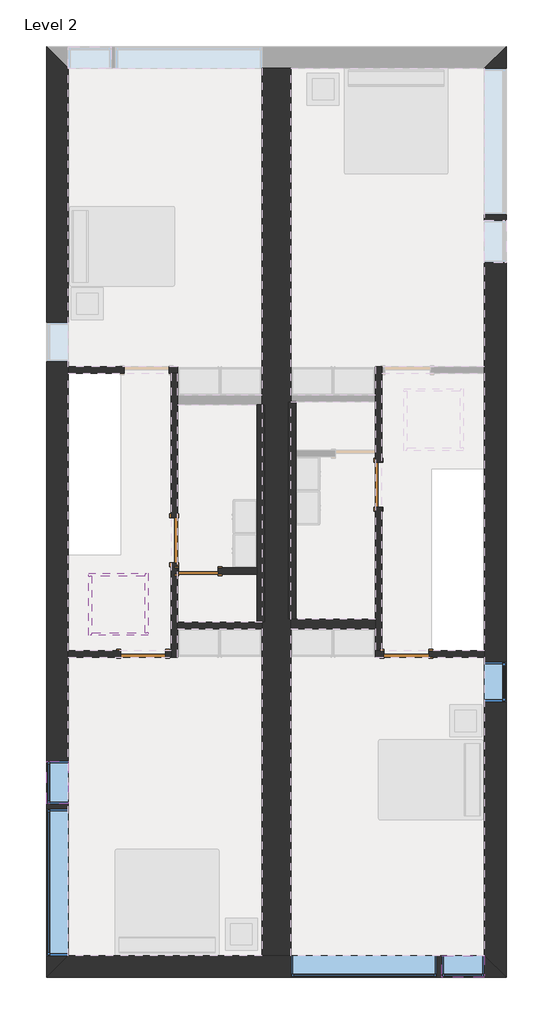
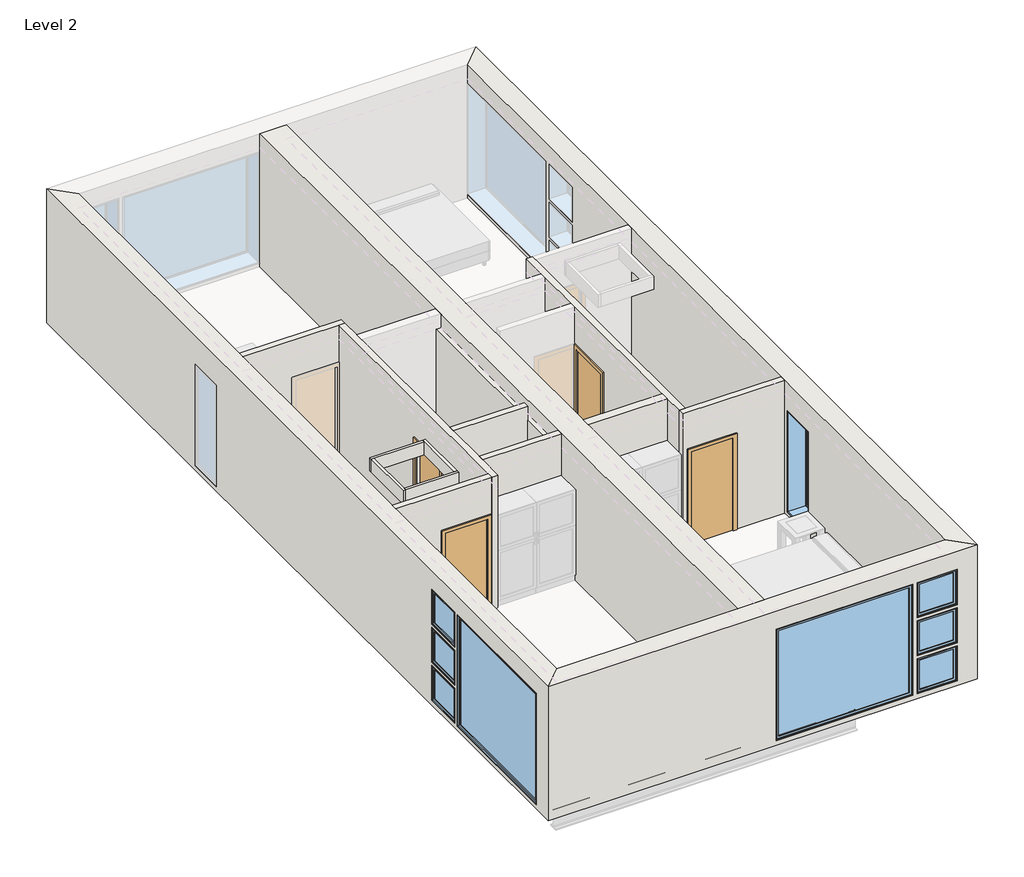
# One storey, part 1 of 2: 20 walls, 9 windows, 5 doors.
# Revit data of these elements (continued)
# Type "Interior - Partition (92mm Stud)" (continued)
#   Constituents = "Constituents"
#   Features = "Features"
#   Finish = "Finish"
#   Grade = "Grade"
#   Material = "Material"
#   ModelReference = "ModelReference"
#   NominalHeight = "NominalHeight"
#   NominalLength = "NominalLength"
#   NominalWidth = "NominalWidth"
#   ProductionYear = "ProductionYear"
#   Reference = "Reference"
#   Shape = "Shape"
#   Size = "Size"
#   SustainabilityPerformance = "SustainabilityPerformance"
#   WarrantyDescription = "WarrantyDescription"
#   WarrantyDurationLabor = "WarrantyDurationLabor"
#   WarrantyDurationParts = "WarrantyDurationParts"
#   WarrantyGuarantorLabor = "WarrantyGuarantorLabor"
#   WarrantyGuarantorParts = "WarrantyGuarantorParts"
#   ExpectedLife = "ExpectedLife"
#   ReplacementCost = "ReplacementCost"
#   AssetAccountingType = "FIXED"
#   Classification Description = "Metal-Framed Gypsum Board Fixed Partitions"
#   Classification Code = "23-25 40 11 11 11"
#   ModelLabel = "ModelLabel"
#   Layers, outside or top first: 0.016 m "Plasterboard" (function 5); 0.092 m "Metal - Stud Layer" (function 1); 0.016 m "Plasterboard" (function 5)
# Type "Interior - Plumbing (152mm Stud)"
#   Manufacturer = "Manufacturer"
#   AccessibilityPerformance = "AccessibilityPerformance"
#   CodePerformance = "CodePerformance"
#   Color = "Color"
#   Constituents = "Constituents"
#   Features = "Features"
#   Finish = "Finish"
#   Grade = "Grade"
#   Material = "Material"
#   ModelReference = "ModelReference"
#   NominalHeight = "NominalHeight"
#   NominalLength = "NominalLength"
#   NominalWidth = "NominalWidth"
#   ProductionYear = "ProductionYear"
#   Reference = "Reference"
#   Shape = "Shape"
#   Size = "Size"
#   SustainabilityPerformance = "SustainabilityPerformance"
#   WarrantyDescription = "WarrantyDescription"
#   WarrantyDurationLabor = "WarrantyDurationLabor"
#   WarrantyDurationParts = "WarrantyDurationParts"
#   WarrantyGuarantorLabor = "WarrantyGuarantorLabor"
#   WarrantyGuarantorParts = "WarrantyGuarantorParts"
#   ExpectedLife = "ExpectedLife"
#   ReplacementCost = "ReplacementCost"
#   AssetAccountingType = "FIXED"
#   Classification Description = "Metal-Framed Gypsum Board Fixed Partitions"
#   Classification Code = "23-25 40 11 11 11"
#   ModelLabel = "ModelLabel"
#   Layers, outside or top first: 0.016 m "Plasterboard" (function 5); 0.152 m "Metal - Stud Layer" (function 1); 0.016 m "Plasterboard" (function 5)
# Type "M_Casement : 819mm x 759mm"
#   Manufacturer = "Manufacturer"
#   Type Mark = "03"
#   Construction Type = "Construction Type"
#   AccessibilityPerformance = "AccessibilityPerformance"
#   CodePerformance = "CodePerformance"
#   ConfigurationType = "ConfigurationType"
#   ConstructionType = "ConstructionType"
#   FireRating = "FireRating"
#   GlazingAreaFraction = "GlazingAreaFraction"
#   OperationType = "OperationType"
#   Area = "Area"
#   Color = "Color"
#   Constituents = "Constituents"
#   Features = "Features"
#   Finish = "Finish"
#   Grade = "Grade"
#   Material = "Material"
#   ModelReference = "ModelReference"
#   NominalHeight = "NominalHeight"
#   NominalLength = "NominalLength"
#   NominalWidth = "NominalWidth"
#   ProductionYear = "ProductionYear"
#   Reference = "Reference"
#   Shape = "Shape"
#   Size = "Size"
#   SustainabilityPerformance = "SustainabilityPerformance"
#   WarrantyDescription = "WarrantyDescription"
#   WarrantyDurationLabor = "WarrantyDurationLabor"
#   WarrantyDurationParts = "WarrantyDurationParts"
#   WarrantyGuarantorLabor = "WarrantyGuarantorLabor"
#   WarrantyGuarantorParts = "WarrantyGuarantorParts"
#   ExpectedLife = "ExpectedLife"
#   ReplacementCost = "ReplacementCost"
#   AssetAccountingType = "FIXED"
#   ModelLabel = "ModelLabel"
#   Height = 0.759 m
#   Default Sill Height = 0.915 m
#   Width = 0.819 m
#   Window Inset = 0.019 m
#   Glass Pane Material = Glass
#   Sash = Sash
#   Trim Exterior Material = Trim
#   Trim Interior Material = Trim
#   Wall Closure = (empty or 0)
# Type "M_Fixed : 2800mm x 2410mm"
#   Manufacturer = "Manufacturer"
#   Type Mark = "01"
#   Construction Type = "Construction Type"
#   AccessibilityPerformance = "AccessibilityPerformance"
#   CodePerformance = "CodePerformance"
#   ConfigurationType = "ConfigurationType"
#   ConstructionType = "ConstructionType"
#   FireRating = "FireRating"
#   GlazingAreaFraction = "GlazingAreaFraction"
#   OperationType = "OperationType"
#   Area = "Area"
#   Color = "Color"
#   Constituents = "Constituents"
#   Features = "Features"
#   Finish = "Finish"
#   Grade = "Grade"
#   Material = "Material"
#   ModelReference = "ModelReference"
#   NominalHeight = "NominalHeight"
#   NominalLength = "NominalLength"
#   NominalWidth = "NominalWidth"
#   ProductionYear = "ProductionYear"
#   Reference = "Reference"
#   Shape = "Shape"
#   Size = "Size"
#   SustainabilityPerformance = "SustainabilityPerformance"
#   WarrantyDescription = "WarrantyDescription"
#   WarrantyDurationLabor = "WarrantyDurationLabor"
#   WarrantyDurationParts = "WarrantyDurationParts"
#   WarrantyGuarantorLabor = "WarrantyGuarantorLabor"
#   WarrantyGuarantorParts = "WarrantyGuarantorParts"
#   ExpectedLife = "ExpectedLife"
#   ReplacementCost = "ReplacementCost"
#   AssetAccountingType = "FIXED"
#   ModelLabel = "ModelLabel"
#   Height = 2.410 m
#   Default Sill Height = 0.100 m
#   Width = 2.800 m
#   Window Inset = 0.019 m
#   Frame Exterior Material = Sash
#   Frame Interior Material = Sash
#   Glass Pane Material = Glass
#   Sash = Sash
#   Wall Closure = (empty or 0)
# Type "M_Fixed : 750mm x 2200mm"
#   Manufacturer = "Manufacturer"
#   Type Mark = "04"
#   Construction Type = "Construction Type"
#   AccessibilityPerformance = "AccessibilityPerformance"
#   CodePerformance = "CodePerformance"
#   ConfigurationType = "ConfigurationType"
#   ConstructionType = "ConstructionType"
#   FireRating = "FireRating"
#   GlazingAreaFraction = "GlazingAreaFraction"
#   OperationType = "OperationType"
#   Area = "Area"
#   Color = "Color"
#   Constituents = "Constituents"
#   Features = "Features"
#   Finish = "Finish"
#   Grade = "Grade"
#   Material = "Material"
#   ModelReference = "ModelReference"
#   NominalHeight = "NominalHeight"
#   NominalLength = "NominalLength"
#   NominalWidth = "NominalWidth"
#   ProductionYear = "ProductionYear"
#   Reference = "Reference"
#   Shape = "Shape"
#   Size = "Size"
#   SustainabilityPerformance = "SustainabilityPerformance"
#   WarrantyDescription = "WarrantyDescription"
#   WarrantyDurationLabor = "WarrantyDurationLabor"
#   WarrantyDurationParts = "WarrantyDurationParts"
#   WarrantyGuarantorLabor = "WarrantyGuarantorLabor"
#   WarrantyGuarantorParts = "WarrantyGuarantorParts"
#   ExpectedLife = "ExpectedLife"
#   ReplacementCost = "ReplacementCost"
#   AssetAccountingType = "FIXED"
#   ModelLabel = "ModelLabel"
#   Height = 2.200 m
#   Default Sill Height = 0.100 m
#   Width = 0.750 m
#   Window Inset = 0.019 m
#   Frame Exterior Material = Sash
#   Frame Interior Material = Sash
#   Glass Pane Material = Glass
#   Sash = Sash
#   Wall Closure = (empty or 0)
# Type "M_Fixed : 819mm x 759mm"
#   Manufacturer = "Manufacturer"
#   Type Mark = "02"
#   Construction Type = "Construction Type"
#   AccessibilityPerformance = "AccessibilityPerformance"
#   CodePerformance = "CodePerformance"
#   ConfigurationType = "ConfigurationType"
#   ConstructionType = "ConstructionType"
#   FireRating = "FireRating"
#   GlazingAreaFraction = "GlazingAreaFraction"
#   OperationType = "OperationType"
#   Area = "Area"
#   Color = "Color"
#   Constituents = "Constituents"
#   Features = "Features"
#   Finish = "Finish"
#   Grade = "Grade"
#   Material = "Material"
#   ModelReference = "ModelReference"
#   NominalHeight = "NominalHeight"
#   NominalLength = "NominalLength"
#   NominalWidth = "NominalWidth"
#   ProductionYear = "ProductionYear"
#   Reference = "Reference"
#   Shape = "Shape"
#   Size = "Size"
#   SustainabilityPerformance = "SustainabilityPerformance"
#   WarrantyDescription = "WarrantyDescription"
#   WarrantyDurationLabor = "WarrantyDurationLabor"
#   WarrantyDurationParts = "WarrantyDurationParts"
#   WarrantyGuarantorLabor = "WarrantyGuarantorLabor"
#   WarrantyGuarantorParts = "WarrantyGuarantorParts"
#   ExpectedLife = "ExpectedLife"
#   ReplacementCost = "ReplacementCost"
#   AssetAccountingType = "FIXED"
#   ModelLabel = "ModelLabel"
#   Height = 0.759 m
#   Default Sill Height = 0.100 m
#   Width = 0.819 m
#   Window Inset = 0.019 m
#   Frame Exterior Material = Sash
#   Frame Interior Material = Sash
#   Glass Pane Material = Glass
#   Sash = Sash
#   Wall Closure = (empty or 0)
# Element 1 (IfcDoor, "M_Single-Flush : 0762 x 2032mm")
#   InstallationDate = "InstallationDate"
#   SerialNumber = "SerialNumber"
#   WarrantyStartDate = "WarrantyStartDate"
#   BarCode = "BarCode"
#   AssetIdentifier = "AssetIdentifier"
#   TagNumber = "TagNumber"
#   URI = "https://niras.dk/projects/0001/door_1xS3BCk291UvhgP2dvNd%24j"
#   Phase Created = New Construction
#   Materials on its faces: "Door - Frame", "Door - Panel"
# Element 2 (IfcDoor, "M_Single-Flush : 0864 x 2032mm")
#   InstallationDate = "InstallationDate"
#   SerialNumber = "SerialNumber"
#   WarrantyStartDate = "WarrantyStartDate"
#   BarCode = "BarCode"
#   AssetIdentifier = "AssetIdentifier"
#   TagNumber = "TagNumber"
#   URI = "https://niras.dk/projects/0001/door_1xS3BCk291UvhgP2dvNo%24h"
#   Phase Created = New Construction
#   Materials on its faces: "Door - Frame", "Door - Panel"
# Element 3 (IfcDoor, "M_Single-Flush : 0864 x 2032mm")
#   InstallationDate = "InstallationDate"
#   SerialNumber = "SerialNumber"
#   WarrantyStartDate = "WarrantyStartDate"
#   BarCode = "BarCode"
#   AssetIdentifier = "AssetIdentifier"
#   TagNumber = "TagNumber"
#   URI = "https://niras.dk/projects/0001/door_1xS3BCk291UvhgP2dvNnLa"
#   Phase Created = New Construction
#   Materials on its faces: "Door - Frame", "Door - Panel"
# Element 4 (IfcDoor, "M_Single-Flush : 0864 x 2032mm")
#   InstallationDate = "InstallationDate"
#   SerialNumber = "SerialNumber"
#   WarrantyStartDate = "WarrantyStartDate"
#   BarCode = "BarCode"
#   AssetIdentifier = "AssetIdentifier"
#   TagNumber = "TagNumber"
#   URI = "https://niras.dk/projects/0001/door_1xS3BCk291UvhgP2dvNnNr"
#   Phase Created = New Construction
#   Materials on its faces: "Door - Frame", "Door - Panel"
# Element 5 (IfcDoor, "M_Single-Flush : 0864 x 2032mm")
#   InstallationDate = "InstallationDate"
#   SerialNumber = "SerialNumber"
#   WarrantyStartDate = "WarrantyStartDate"
#   BarCode = "BarCode"
#   AssetIdentifier = "AssetIdentifier"
#   TagNumber = "TagNumber"
#   URI = "https://niras.dk/projects/0001/door_1xS3BCk291UvhgP2dvNmlJ"
#   Phase Created = New Construction
#   Materials on its faces: "Door - Frame", "Door - Panel"
# Element 6 (IfcWall, "Party Wall - CMU Residential Unit Dimising Wall")
#   InstallationDate = "InstallationDate"
#   SerialNumber = "SerialNumber"
#   WarrantyStartDate = "WarrantyStartDate"
#   BarCode = "BarCode"
#   AssetIdentifier = "AssetIdentifier"
#   TagNumber = "TagNumber"
#   URI = "https://niras.dk/projects/0001/wall_1xS3BCk291UvhgP2dvNqkY"
#   Top Offset = 0.000 m
#   Base Offset = 0.000 m
#   wall height = 2.900 m
#   Phase Created = New Construction
#   Base Constraint = Level 2
#   Top Constraint = Roof
#   Materials on its faces: "Default Wall", "Plasterboard"
# Element 7 (IfcWall, "Exterior - Brick on Block")
#   InstallationDate = "InstallationDate"
#   SerialNumber = "SerialNumber"
#   WarrantyStartDate = "WarrantyStartDate"
#   BarCode = "BarCode"
#   AssetIdentifier = "AssetIdentifier"
#   TagNumber = "TagNumber"
#   URI = "https://niras.dk/projects/0001/wall_1xS3BCk291UvhgP2dvNrHJ"
#   Top Offset = 0.000 m
#   Base Offset = 0.000 m
#   wall height = 2.900 m
#   Phase Created = New Construction
#   Base Constraint = Level 2
#   Top Constraint = Roof
#   Materials on its faces: "Default Wall", "Plasterboard", "Masonry - Brick"
# Element 8 (IfcWall, "Exterior - Brick on Block")
#   InstallationDate = "InstallationDate"
#   SerialNumber = "SerialNumber"
#   WarrantyStartDate = "WarrantyStartDate"
#   BarCode = "BarCode"
#   AssetIdentifier = "AssetIdentifier"
#   TagNumber = "TagNumber"
#   URI = "https://niras.dk/projects/0001/wall_1xS3BCk291UvhgP2dvNrIB"
#   Top Offset = 0.000 m
#   Base Offset = 0.000 m
#   wall height = 2.900 m
#   Phase Created = New Construction
#   Base Constraint = Level 2
#   Top Constraint = Roof
#   Materials on its faces: "Default Wall", "Plasterboard", "Masonry - Brick"
# Element 9 (IfcWall, "Exterior - Brick on Block")
#   InstallationDate = "InstallationDate"
#   SerialNumber = "SerialNumber"
#   WarrantyStartDate = "WarrantyStartDate"
#   BarCode = "BarCode"
#   AssetIdentifier = "AssetIdentifier"
#   TagNumber = "TagNumber"
#   URI = "https://niras.dk/projects/0001/wall_1xS3BCk291UvhgP2dvNrJ3"
#   Top Offset = 0.000 m
#   Base Offset = 0.000 m
#   wall height = 2.900 m
#   Phase Created = New Construction
#   Base Constraint = Level 2
#   Top Constraint = Roof
#   Materials on its faces: "Default Wall", "Plasterboard", "Masonry - Brick"
# Element 10 (IfcWall, "Interior - Furring (152 mm Stud)")
#   InstallationDate = "InstallationDate"
#   SerialNumber = "SerialNumber"
#   WarrantyStartDate = "WarrantyStartDate"
#   BarCode = "BarCode"
#   AssetIdentifier = "AssetIdentifier"
#   TagNumber = "TagNumber"
#   URI = "https://niras.dk/projects/0001/wall_1xS3BCk291UvhgP2dvNvRw"
#   Top Offset = -0.305 m
#   Base Offset = 0.000 m
#   wall height = 2.595 m
#   Phase Created = New Construction
#   Base Constraint = Level 2
#   Top Constraint = Roof
#   Materials on its faces: "Default Wall", "Metal - Stud Layer", "Plasterboard"
# Element 11 (IfcWall, "Interior - Furring (152 mm Stud)")
#   InstallationDate = "InstallationDate"
#   SerialNumber = "SerialNumber"
#   WarrantyStartDate = "WarrantyStartDate"
#   BarCode = "BarCode"
#   AssetIdentifier = "AssetIdentifier"
#   TagNumber = "TagNumber"
#   URI = "https://niras.dk/projects/0001/wall_1xS3BCk291UvhgP2dvNv9J"
#   Top Offset = -0.305 m
#   Base Offset = 0.000 m
#   wall height = 2.595 m
#   Phase Created = New Construction
#   Base Constraint = Level 2
#   Top Constraint = Roof
#   Materials on its faces: "Default Wall", "Metal - Stud Layer", "Plasterboard"
# Element 12 (IfcWall, "Interior - Furring (38 mm Stud)")
#   InstallationDate = "InstallationDate"
#   SerialNumber = "SerialNumber"
#   WarrantyStartDate = "WarrantyStartDate"
#   BarCode = "BarCode"
#   AssetIdentifier = "AssetIdentifier"
#   TagNumber = "TagNumber"
#   URI = "https://niras.dk/projects/0001/wall_1xS3BCk291UvhgP2dvNZNC"
#   built-in parameter 1001111 = 2.612 m
#   Top Offset = 0.000 m
#   Base Offset = 2.612 m
#   wall height = 0.288 m
#   Phase Created = New Construction
#   Base Constraint = Level 2
#   Top Constraint = Roof
#   Materials on its faces: "Default Wall", "Metal - Stud Layer", "Plasterboard"
# Element 13 (IfcWall, "Interior - Furring (38 mm Stud)")
#   InstallationDate = "InstallationDate"
#   SerialNumber = "SerialNumber"
#   WarrantyStartDate = "WarrantyStartDate"
#   BarCode = "BarCode"
#   AssetIdentifier = "AssetIdentifier"
#   TagNumber = "TagNumber"
#   URI = "https://niras.dk/projects/0001/wall_1xS3BCk291UvhgP2dvNZNF"
#   built-in parameter 1001111 = 2.612 m
#   Top Offset = 0.000 m
#   Base Offset = 2.612 m
#   wall height = 0.288 m
#   Phase Created = New Construction
#   Base Constraint = Level 2
#   Top Constraint = Roof
#   Materials on its faces: "Default Wall", "Metal - Stud Layer", "Plasterboard"
# Element 14 (IfcWall, "Interior - Furring (38 mm Stud)")
#   InstallationDate = "InstallationDate"
#   SerialNumber = "SerialNumber"
#   WarrantyStartDate = "WarrantyStartDate"
#   BarCode = "BarCode"
#   AssetIdentifier = "AssetIdentifier"
#   TagNumber = "TagNumber"
#   URI = "https://niras.dk/projects/0001/wall_1xS3BCk291UvhgP2dvNZNE"
#   built-in parameter 1001111 = 2.612 m
#   Top Offset = 0.000 m
#   Base Offset = 2.612 m
#   wall height = 0.288 m
#   Phase Created = New Construction
#   Base Constraint = Level 2
#   Top Constraint = Roof
#   Materials on its faces: "Default Wall", "Metal - Stud Layer", "Plasterboard"
# Element 15 (IfcWall, "Interior - Furring (38 mm Stud)")
#   InstallationDate = "InstallationDate"
#   SerialNumber = "SerialNumber"
#   WarrantyStartDate = "WarrantyStartDate"
#   BarCode = "BarCode"
#   AssetIdentifier = "AssetIdentifier"
#   TagNumber = "TagNumber"
#   URI = "https://niras.dk/projects/0001/wall_1xS3BCk291UvhgP2dvNZN9"
#   built-in parameter 1001111 = 2.612 m
#   Top Offset = 0.000 m
#   Base Offset = 2.612 m
#   wall height = 0.288 m
#   Phase Created = New Construction
#   Base Constraint = Level 2
#   Top Constraint = Roof
#   Materials on its faces: "Default Wall", "Metal - Stud Layer", "Plasterboard"
# Element 16 (IfcWall, "Interior - Partition (92mm Stud)")
#   InstallationDate = "InstallationDate"
#   SerialNumber = "SerialNumber"
#   WarrantyStartDate = "WarrantyStartDate"
#   BarCode = "BarCode"
#   AssetIdentifier = "AssetIdentifier"
#   TagNumber = "TagNumber"
#   URI = "https://niras.dk/projects/0001/wall_1xS3BCk291UvhgP2dvNrNL"
#   built-in parameter 1001111 = -0.488 m
#   Top Offset = 0.000 m
#   Base Offset = -0.488 m
#   wall height = 3.388 m
#   Phase Created = New Construction
#   Base Constraint = Level 2
#   Top Constraint = Roof
#   Materials on its faces: "Plasterboard"
# Element 17 (IfcWall, "Interior - Partition (92mm Stud)")
#   InstallationDate = "InstallationDate"
#   SerialNumber = "SerialNumber"
#   WarrantyStartDate = "WarrantyStartDate"
#   BarCode = "BarCode"
#   AssetIdentifier = "AssetIdentifier"
#   TagNumber = "TagNumber"
#   URI = "https://niras.dk/projects/0001/wall_1xS3BCk291UvhgP2dvNrOK"
#   Top Offset = 0.000 m
#   Base Offset = 0.000 m
#   wall height = 2.900 m
#   Phase Created = New Construction
#   Base Constraint = Level 2
#   Top Constraint = Roof
#   Materials on its faces: "Plasterboard"
# Element 18 (IfcWall, "Interior - Partition (92mm Stud)")
#   InstallationDate = "InstallationDate"
#   SerialNumber = "SerialNumber"
#   WarrantyStartDate = "WarrantyStartDate"
#   BarCode = "BarCode"
#   AssetIdentifier = "AssetIdentifier"
#   TagNumber = "TagNumber"
#   URI = "https://niras.dk/projects/0001/wall_1xS3BCk291UvhgP2dvNrPz"
#   Top Offset = 0.000 m
#   Base Offset = 0.000 m
#   wall height = 2.900 m
#   Phase Created = New Construction
#   Base Constraint = Level 2
#   Top Constraint = Roof
#   Materials on its faces: "Plasterboard"
# Element 19 (IfcWall, "Interior - Partition (92mm Stud)")
#   InstallationDate = "InstallationDate"
#   SerialNumber = "SerialNumber"
#   WarrantyStartDate = "WarrantyStartDate"
#   BarCode = "BarCode"
#   AssetIdentifier = "AssetIdentifier"
#   TagNumber = "TagNumber"
#   URI = "https://niras.dk/projects/0001/wall_1xS3BCk291UvhgP2dvNrU8"
#   Top Offset = 0.000 m
#   Base Offset = 0.000 m
#   wall height = 2.900 m
#   Phase Created = New Construction
#   Base Constraint = Level 2
#   Top Constraint = Roof
#   Materials on its faces: "Plasterboard"
# Element 20 (IfcWall, "Interior - Partition (92mm Stud)")
#   InstallationDate = "InstallationDate"
#   SerialNumber = "SerialNumber"
#   WarrantyStartDate = "WarrantyStartDate"
#   BarCode = "BarCode"
#   AssetIdentifier = "AssetIdentifier"
#   TagNumber = "TagNumber"
#   URI = "https://niras.dk/projects/0001/wall_1xS3BCk291UvhgP2dvNr2Z"
#   built-in parameter 1001111 = -0.488 m
#   Top Offset = 0.000 m
#   Base Offset = -0.488 m
#   wall height = 3.388 m
#   Phase Created = New Construction
#   Base Constraint = Level 2
#   Top Constraint = Roof
#   Materials on its faces: "Plasterboard"
# Element 21 (IfcWall, "Interior - Partition (92mm Stud)")
#   InstallationDate = "InstallationDate"
#   SerialNumber = "SerialNumber"
#   WarrantyStartDate = "WarrantyStartDate"
#   BarCode = "BarCode"
#   AssetIdentifier = "AssetIdentifier"
#   TagNumber = "TagNumber"
#   URI = "https://niras.dk/projects/0001/wall_1xS3BCk291UvhgP2dvNr3l"
#   Top Offset = 0.000 m
#   Base Offset = 0.000 m
#   wall height = 2.900 m
#   Phase Created = New Construction
#   Base Constraint = Level 2
#   Top Constraint = Roof
#   Materials on its faces: "Plasterboard"
# Element 22 (IfcWall, "Interior - Partition (92mm Stud)")
#   InstallationDate = "InstallationDate"
#   SerialNumber = "SerialNumber"
#   WarrantyStartDate = "WarrantyStartDate"
#   BarCode = "BarCode"
#   AssetIdentifier = "AssetIdentifier"
#   TagNumber = "TagNumber"
#   URI = "https://niras.dk/projects/0001/wall_1xS3BCk291UvhgP2dvNdvs"
#   Top Offset = 0.000 m
#   Base Offset = 0.000 m
#   wall height = 2.900 m
#   Phase Created = New Construction
#   Base Constraint = Level 2
#   Top Constraint = Roof
#   Materials on its faces: "Plasterboard"
# Element 23 (IfcWall, "Interior - Partition (92mm Stud)")
#   InstallationDate = "InstallationDate"
#   SerialNumber = "SerialNumber"
#   WarrantyStartDate = "WarrantyStartDate"
#   BarCode = "BarCode"
#   AssetIdentifier = "AssetIdentifier"
#   TagNumber = "TagNumber"
#   URI = "https://niras.dk/projects/0001/wall_1xS3BCk291UvhgP2dvNdef"
#   built-in parameter 1001111 = -0.488 m
#   Top Offset = 0.000 m
#   Base Offset = -0.488 m
#   wall height = 0.488 m
#   Phase Created = New Construction
#   Base Constraint = Level 2
#   Top Constraint = Level 2
#   Materials on its faces: "Plasterboard"
# Element 24 (IfcWall, "Interior - Partition (92mm Stud)")
#   InstallationDate = "InstallationDate"
#   SerialNumber = "SerialNumber"
#   WarrantyStartDate = "WarrantyStartDate"
#   BarCode = "BarCode"
#   AssetIdentifier = "AssetIdentifier"
#   TagNumber = "TagNumber"
#   URI = "https://niras.dk/projects/0001/wall_1xS3BCk291UvhgP2dvNdhe"
#   built-in parameter 1001111 = -0.488 m
#   Top Offset = 0.000 m
#   Base Offset = -0.488 m
#   wall height = 0.488 m
#   Phase Created = New Construction
#   Base Constraint = Level 2
#   Top Constraint = Level 2
#   Materials on its faces: "Plasterboard"
# Element 25 (IfcWall, "Interior - Plumbing (152mm Stud)")
#   InstallationDate = "InstallationDate"
#   SerialNumber = "SerialNumber"
#   WarrantyStartDate = "WarrantyStartDate"
#   BarCode = "BarCode"
#   AssetIdentifier = "AssetIdentifier"
#   TagNumber = "TagNumber"
#   URI = "https://niras.dk/projects/0001/wall_1xS3BCk291UvhgP2dvNr6g"
#   Top Offset = 0.000 m
#   Base Offset = 0.000 m
#   wall height = 2.900 m
#   Phase Created = New Construction
#   Base Constraint = Level 2
#   Top Constraint = Roof
#   Materials on its faces: "Default Wall", "Plasterboard"
# Element 26 (IfcWindow, "M_Casement : 819mm x 759mm")
#   Mark = "20"
#   InstallationDate = "InstallationDate"
#   SerialNumber = "SerialNumber"
#   WarrantyStartDate = "WarrantyStartDate"
#   BarCode = "BarCode"
#   AssetIdentifier = "AssetIdentifier"
#   TagNumber = "TagNumber"
#   URI = "https://niras.dk/projects/0001/window_1xS3BCk291UvhgP2dvNopD"
#   Phase Created = New Construction
#   Materials on its faces: "Trim", "Sash", "Glass"
# Element 27 (IfcWindow, "M_Casement : 819mm x 759mm")
#   Mark = "25"
#   InstallationDate = "InstallationDate"
#   SerialNumber = "SerialNumber"
#   WarrantyStartDate = "WarrantyStartDate"
#   BarCode = "BarCode"
#   AssetIdentifier = "AssetIdentifier"
#   TagNumber = "TagNumber"
#   URI = "https://niras.dk/projects/0001/window_1xS3BCk291UvhgP2dvNwSd"
#   Phase Created = New Construction
#   Materials on its faces: "Trim", "Sash", "Glass"
# Element 28 (IfcWindow, "M_Fixed : 2800mm x 2410mm")
#   Mark = "18"
#   InstallationDate = "InstallationDate"
#   SerialNumber = "SerialNumber"
#   WarrantyStartDate = "WarrantyStartDate"
#   BarCode = "BarCode"
#   AssetIdentifier = "AssetIdentifier"
#   TagNumber = "TagNumber"
#   URI = "https://niras.dk/projects/0001/window_1xS3BCk291UvhgP2dvNoCx"
#   Phase Created = New Construction
#   Materials on its faces: "Sash", "Glass"
# Element 29 (IfcWindow, "M_Fixed : 2800mm x 2410mm")
#   Mark = "22"
#   InstallationDate = "InstallationDate"
#   SerialNumber = "SerialNumber"
#   WarrantyStartDate = "WarrantyStartDate"
#   BarCode = "BarCode"
#   AssetIdentifier = "AssetIdentifier"
#   TagNumber = "TagNumber"
#   URI = "https://niras.dk/projects/0001/window_1xS3BCk291UvhgP2dvNwHx"
#   Phase Created = New Construction
#   Materials on its faces: "Sash", "Glass"
# Element 30 (IfcWindow, "M_Fixed : 750mm x 2200mm")
#   Mark = "31"
#   InstallationDate = "InstallationDate"
#   SerialNumber = "SerialNumber"
#   WarrantyStartDate = "WarrantyStartDate"
#   BarCode = "BarCode"
#   AssetIdentifier = "AssetIdentifier"
#   TagNumber = "TagNumber"
#   URI = "https://niras.dk/projects/0001/window_1xS3BCk291UvhgP2dvNwAF"
#   Phase Created = New Construction
#   Materials on its faces: "Sash", "Glass"
# Element 31 (IfcWindow, "M_Fixed : 819mm x 759mm")
#   Mark = "19"
#   InstallationDate = "InstallationDate"
#   SerialNumber = "SerialNumber"
#   WarrantyStartDate = "WarrantyStartDate"
#   BarCode = "BarCode"
#   AssetIdentifier = "AssetIdentifier"
#   TagNumber = "TagNumber"
#   URI = "https://niras.dk/projects/0001/window_1xS3BCk291UvhgP2dvNom4"
#   Phase Created = New Construction
#   Materials on its faces: "Sash", "Glass"
# Element 32 (IfcWindow, "M_Fixed : 819mm x 759mm")
#   Mark = "21"
#   InstallationDate = "InstallationDate"
#   SerialNumber = "SerialNumber"
#   WarrantyStartDate = "WarrantyStartDate"
#   BarCode = "BarCode"
#   AssetIdentifier = "AssetIdentifier"
#   TagNumber = "TagNumber"
#   URI = "https://niras.dk/projects/0001/window_1xS3BCk291UvhgP2dvNos1"
#   Phase Created = New Construction
#   Materials on its faces: "Sash", "Glass"
# Element 33 (IfcWindow, "M_Fixed : 819mm x 759mm")
#   Mark = "23"
#   InstallationDate = "InstallationDate"
#   SerialNumber = "SerialNumber"
#   WarrantyStartDate = "WarrantyStartDate"
#   BarCode = "BarCode"
#   AssetIdentifier = "AssetIdentifier"
#   TagNumber = "TagNumber"
#   URI = "https://niras.dk/projects/0001/window_1xS3BCk291UvhgP2dvNwMI"
#   Phase Created = New Construction
#   Materials on its faces: "Sash", "Glass"
# Element 34 (IfcWindow, "M_Fixed : 819mm x 759mm")
#   Mark = "24"
#   InstallationDate = "InstallationDate"
#   SerialNumber = "SerialNumber"
#   WarrantyStartDate = "WarrantyStartDate"
#   BarCode = "BarCode"
#   AssetIdentifier = "AssetIdentifier"
#   TagNumber = "TagNumber"
#   URI = "https://niras.dk/projects/0001/window_1xS3BCk291UvhgP2dvNwQb"
#   Phase Created = New Construction
#   Materials on its faces: "Sash", "Glass"
# Materials
#   "Door - Panel": class "Wood", colour RGB 210 159 95, transparency 0
#   "Door - Frame": class "Miscellaneous", colour RGB 118 70 51, transparency 0
#   "Plasterboard": class "Drywall", colour RGB 249 249 249, transparency 0, Description = "Interior finish"
#   "Metal - Stud Layer": class "Metal", colour RGB 127 127 127, transparency 0
#   "Masonry - Concrete Block": class "Concrete", colour RGB 181 181 181, transparency 0
#   "Misc. Air Layers - Air Space": class "Miscellaneous", colour RGB 255 255 255, transparency 0
#   "Masonry - Brick": class "Brick", colour RGB 170 100 105, transparency 0, Cost = 0
#   "Air Barrier - Air Infiltration Barrier": class "Miscellaneous", colour RGB 127 127 127, transparency 0
#   "Insulation / Thermal Barriers - Rigid insulation": class "Miscellaneous", colour RGB 127 127 127, transparency 0
#   "Vapour / Moisture Barriers - Vapour Retarder": class "Miscellaneous", colour RGB 127 127 127, transparency 0
#   "Glass": class "Glass", colour RGB 0 128 192, transparency 0.9
#   "Sash": class "Wood", colour RGB 224 178 126, transparency 0
#   "Trim": class "Wood", colour RGB 224 178 126, transparency 0
#   "Default Wall": class "Miscellaneous", colour RGB 128 128 128, transparency 0
# Room at (5504.462, -7362.691) mm, phase "New Construction", upper level "Level 2", upper offset 2.600 m, lower offset 0.000 m
#   Number = "A205"
#   Name = "Utility"
#   CeilingCovering = "CeilingCovering"
#   FloorCovering = "FloorCovering"
#   WallCovering = "WallCovering"
#   LoadCapacity = "LoadCapacity"
#   CirculationZoneName = "Unit A CirculationZoneName"
#   FireAlarmZoneName = "Unit A FireAlarmZoneName"
#   HistoricPreservationZoneName = "Unit A HistoricPreservationZoneName"
#   LightingZoneName = "Unit A LightingZoneName"
#   OccupancyZoneName = "Unit A OccupancyZoneName"
#   VentilationZoneName = "Unit A VentilationZoneName"
#   RoomTag = "RoomTag"
#   URI = "https://niras.dk/projects/0001/room_1xS3BCk291UvhgP2dvNdjF"
#   OmniClass Table 13 Category = 13-81 31: Service Distribution Spaces
# Room at (3212.998, -10631.708) mm, phase "New Construction", upper level "Level 2", upper offset 2.600 m, lower offset 0.000 m
#   Number = "B205"
#   Name = "Utility"
#   CeilingCovering = "CeilingCovering"
#   FloorCovering = "FloorCovering"
#   WallCovering = "WallCovering"
#   LoadCapacity = "LoadCapacity"
#   CirculationZoneName = "Unit B CirculationZoneName"
#   FireAlarmZoneName = "Unit B FireAlarmZoneName"
#   HistoricPreservationZoneName = "Unit B HistoricPreservationZoneName"
#   LightingZoneName = "Unit B LightingZoneName"
#   OccupancyZoneName = "Unit B OccupancyZoneName"
#   VentilationZoneName = "Unit B VentilationZoneName"
#   RoomTag = "RoomTag"
#   URI = "https://niras.dk/projects/0001/room_1xS3BCk291UvhgP2dvNdjS"
#   OmniClass Table 13 Category = 13-81 31: Service Distribution Spaces
# Room at (1454.488, -10303.161) mm, phase "New Construction", upper level "Roof", upper offset 0.000 m, lower offset 0.000 m
#   Number = "B201"
#   Name = "Hallway"
#   CeilingCovering = "CeilingCovering"
#   FloorCovering = "FloorCovering"
#   WallCovering = "WallCovering"
#   LoadCapacity = "LoadCapacity"
#   CirculationZoneName = "Unit B CirculationZoneName"
#   FireAlarmZoneName = "Unit B FireAlarmZoneName"
#   HistoricPreservationZoneName = "Unit B HistoricPreservationZoneName"
#   LightingZoneName = "Unit B LightingZoneName"
#   OccupancyZoneName = "Unit B OccupancyZoneName"
#   VentilationZoneName = "Unit B VentilationZoneName"
#   RoomTag = "RoomTag"
#   URI = "https://niras.dk/projects/0001/room_1xS3BCk291UvhgP2dvNcOe"
#   OmniClass Table 13 Category = 13-51 24 11: General Residential Space
# Room at (3089.488, -8171.398) mm, phase "New Construction", upper level "Level 2", upper offset 2.600 m, lower offset 0.000 m
#   Number = "B204"
#   Name = "Bathroom 2"
#   CeilingCovering = "CeilingCovering"
#   FloorCovering = "FloorCovering"
#   WallCovering = "WallCovering"
#   LoadCapacity = "LoadCapacity"
#   CirculationZoneName = "Unit B CirculationZoneName"
#   FireAlarmZoneName = "Unit B FireAlarmZoneName"
#   HistoricPreservationZoneName = "Unit B HistoricPreservationZoneName"
#   LightingZoneName = "Unit B LightingZoneName"
#   OccupancyZoneName = "Unit B OccupancyZoneName"
#   VentilationZoneName = "Unit B VentilationZoneName"
#   RoomTag = "RoomTag"
#   URI = "https://niras.dk/projects/0001/room_1xS3BCk291UvhgP2dvNcOq"
#   OmniClass Table 13 Category = 13-41 11 14 11: Bathroom
# Room at (2299.214, -3193.083) mm, phase "New Construction", upper level "Level 2", upper offset 2.600 m, lower offset 0.000 m
#   Number = "B203"
#   Name = "Bedroom 2"
#   CeilingCovering = "CeilingCovering"
#   FloorCovering = "FloorCovering"
#   WallCovering = "WallCovering"
#   LoadCapacity = "LoadCapacity"
#   CirculationZoneName = "Unit B CirculationZoneName"
#   FireAlarmZoneName = "Unit B FireAlarmZoneName"
#   HistoricPreservationZoneName = "Unit B HistoricPreservationZoneName"
#   LightingZoneName = "Unit B LightingZoneName"
#   OccupancyZoneName = "Unit B OccupancyZoneName"
#   VentilationZoneName = "Unit B VentilationZoneName"
#   RoomTag = "RoomTag"
#   URI = "https://niras.dk/projects/0001/room_1xS3BCk291UvhgP2dvNcOn"
#   OmniClass Table 13 Category = 13-51 21 11: Bedroom
# Room at (2389.183, -14169.377) mm, phase "New Construction", upper level "Level 2", upper offset 2.600 m, lower offset 0.000 m
#   Number = "B202"
#   Name = "Bedroom 1"
#   CeilingCovering = "CeilingCovering"
#   FloorCovering = "FloorCovering"
#   WallCovering = "WallCovering"
#   LoadCapacity = "LoadCapacity"
#   CirculationZoneName = "Unit B CirculationZoneName"
#   FireAlarmZoneName = "Unit B FireAlarmZoneName"
#   HistoricPreservationZoneName = "Unit B HistoricPreservationZoneName"
#   LightingZoneName = "Unit B LightingZoneName"
#   OccupancyZoneName = "Unit B OccupancyZoneName"
#   VentilationZoneName = "Unit B VentilationZoneName"
#   RoomTag = "RoomTag"
#   URI = "https://niras.dk/projects/0001/room_1xS3BCk291UvhgP2dvNcOo"
#   OmniClass Table 13 Category = 13-51 21 11: Bedroom
# Room at (7422.627, -7362.691) mm, phase "New Construction", upper level "Roof", upper offset 0.000 m, lower offset 0.000 m
#   Number = "A201"
#   Name = "Hallway"
#   CeilingCovering = "CeilingCovering"
#   FloorCovering = "FloorCovering"
#   WallCovering = "WallCovering"
#   LoadCapacity = "LoadCapacity"
#   CirculationZoneName = "Unit A CirculationZoneName"
#   FireAlarmZoneName = "Unit A FireAlarmZoneName"
#   HistoricPreservationZoneName = "Unit A HistoricPreservationZoneName"
#   LightingZoneName = "Unit A LightingZoneName"
#   OccupancyZoneName = "Unit A OccupancyZoneName"
#   VentilationZoneName = "Unit A VentilationZoneName"
#   RoomTag = "RoomTag"
#   URI = "https://niras.dk/projects/0001/room_1xS3BCk291UvhgP2dvNvkK"
#   OmniClass Table 13 Category = 13-51 24 11: General Residential Space
# Room at (5560.258, -8979.154) mm, phase "New Construction", upper level "Level 2", upper offset 2.600 m, lower offset 0.000 m
#   Number = "A204"
#   Name = "Bathroom 2"
#   CeilingCovering = "CeilingCovering"
#   FloorCovering = "FloorCovering"
#   WallCovering = "WallCovering"
#   LoadCapacity = "LoadCapacity"
#   CirculationZoneName = "Unit A CirculationZoneName"
#   FireAlarmZoneName = "Unit A FireAlarmZoneName"
#   HistoricPreservationZoneName = "Unit A HistoricPreservationZoneName"
#   LightingZoneName = "Unit A LightingZoneName"
#   OccupancyZoneName = "Unit A OccupancyZoneName"
#   VentilationZoneName = "Unit A VentilationZoneName"
#   RoomTag = "RoomTag"
#   URI = "https://niras.dk/projects/0001/room_1xS3BCk291UvhgP2dvNvkG"
#   OmniClass Table 13 Category = 13-41 11 14 11: Bathroom
# Room at (6525.931, -14536.263) mm, phase "New Construction", upper level "Level 2", upper offset 2.600 m, lower offset 0.000 m
#   Number = "A203"
#   Name = "Bedroom 2"
#   CeilingCovering = "CeilingCovering"
#   FloorCovering = "FloorCovering"
#   WallCovering = "WallCovering"
#   LoadCapacity = "LoadCapacity"
#   CirculationZoneName = "Unit A CirculationZoneName"
#   FireAlarmZoneName = "Unit A FireAlarmZoneName"
#   HistoricPreservationZoneName = "Unit A HistoricPreservationZoneName"
#   LightingZoneName = "Unit A LightingZoneName"
#   OccupancyZoneName = "Unit A OccupancyZoneName"
#   VentilationZoneName = "Unit A VentilationZoneName"
#   RoomTag = "RoomTag"
#   URI = "https://niras.dk/projects/0001/room_1xS3BCk291UvhgP2dvNvkT"
#   OmniClass Table 13 Category = 13-51 21 11: Bedroom
# Room at (6525.931, -3431.022) mm, phase "New Construction", upper level "Level 2", upper offset 2.600 m, lower offset 0.000 m
#   Number = "A202"
#   Name = "Bedroom 1"
#   CeilingCovering = "CeilingCovering"
#   FloorCovering = "FloorCovering"
#   WallCovering = "WallCovering"
#   LoadCapacity = "LoadCapacity"
#   CirculationZoneName = "Unit A CirculationZoneName"
#   FireAlarmZoneName = "Unit A FireAlarmZoneName"
#   HistoricPreservationZoneName = "Unit A HistoricPreservationZoneName"
#   LightingZoneName = "Unit A LightingZoneName"
#   OccupancyZoneName = "Unit A OccupancyZoneName"
#   VentilationZoneName = "Unit A VentilationZoneName"
#   RoomTag = "RoomTag"
#   URI = "https://niras.dk/projects/0001/room_1xS3BCk291UvhgP2dvNvkU"
#   OmniClass Table 13 Category = 13-51 21 11: Bedroom
